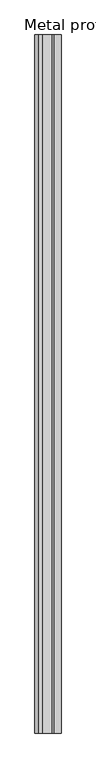
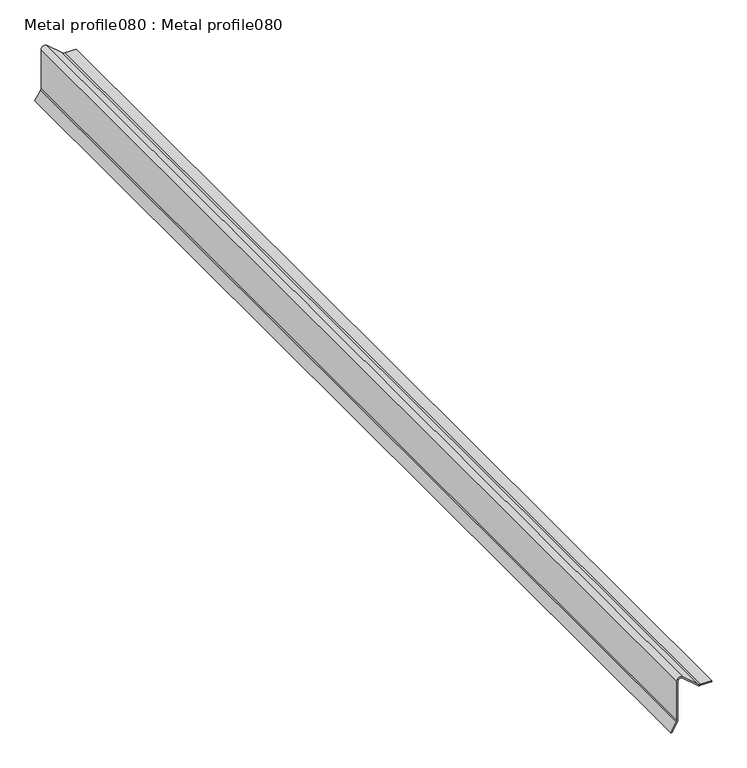
"""IFC4 building model written with IfcOpenShell, lengths in millimetres: proxy geometry, Metal profile080 : Metal profile080."""

from ifc_helpers import new_model, si_unit, point, frame, frame_2d, origin, place, context, project, spatial, polyline, circle_curve, trimmed, segment, composite_curve, outline, extrude, source, transform, mapped, element, save


def metal_profile080_metal_profile080_1098f815(model_context):
    return source(origin(), model_context, "Body", "SweptSolid", [
        extrude(outline(composite_curve([segment(trimmed(circle_curve(frame_2d((40173.6742187, -7212.8179539)), 6.35), [point((40167.3242187, -7212.8179539))], [point((40168.8617194, -7216.9607006))], True, "CARTESIAN"), True, "CONTINUOUS"), segment(polyline([(40168.8617194, -7216.9607006), (40193.006585, -7245.0090359)]), True, "CONTINUOUS"), segment(trimmed(circle_curve(frame_2d((40188.1940856, -7249.1517826)), 6.35), [point((40193.006585, -7245.0090359))], [point((40188.1940856, -7255.5017826))], False, "CARTESIAN"), True, "CONTINUOUS"), segment(polyline([(40188.1940856, -7255.5017826), (40113.9784377, -7255.5017826)]), True, "CONTINUOUS"), segment(trimmed(circle_curve(frame_2d((40113.9784377, -7261.8517826)), 6.35), [point((40113.9784377, -7255.5017826))], [point((40110.6358579, -7256.4527401))], True, "CARTESIAN"), True, "CONTINUOUS"), segment(polyline([(40110.6358579, -7256.4527401), (40093.8632812, -7266.8367435), (40092.8105002, -7265.1362577), (40109.5830768, -7254.7522542)]), True, "CONTINUOUS"), segment(trimmed(circle_curve(frame_2d((40113.9784377, -7261.8517826)), 8.35), [point((40109.5830768, -7254.7522542))], [point((40113.9784377, -7253.5017826))], False, "CARTESIAN"), True, "CONTINUOUS"), segment(polyline([(40113.9784377, -7253.5017826), (40188.1940856, -7253.5017826)]), True, "CONTINUOUS"), segment(trimmed(circle_curve(frame_2d((40188.1940856, -7249.1517826)), 4.35), [point((40188.1940856, -7253.5017826))], [point((40191.4908371, -7246.313838))], True, "CARTESIAN"), True, "CONTINUOUS"), segment(polyline([(40191.4908371, -7246.313838), (40167.3459716, -7218.2655027)]), True, "CONTINUOUS"), segment(trimmed(circle_curve(frame_2d((40173.6742187, -7212.8179539)), 8.35), [point((40167.3459716, -7218.2655027))], [point((40165.3242187, -7212.8179539))], False, "CARTESIAN"), True, "CONTINUOUS"), segment(polyline([(40165.3242187, -7212.8179539), (40165.3242188, -7191.8504154), (40167.3242187, -7191.8504154), (40167.3242187, -7212.8179539)]), True, "CONTINUOUS")], self_intersect=False)), frame((0.0, 7982.1531721, 0.0), z_axis=(0.0, 1.0, 0.0), x_axis=(0.0, 0.0, 1.0)), (0.0, 0.0, 1.0), 2000.0),
    ])


if __name__ == "__main__":
    model = new_model("IFC4")
    model_context = context("Model", 3, world=origin())
    ifc_project = project(units=[si_unit("LENGTHUNIT", "METRE", prefix="MILLI")], contexts=[model_context])
    site = spatial("IfcSite", under=ifc_project)
    building = spatial("IfcBuilding", under=site)
    placement = place(None, origin())
    metal_profile080_metal_profile080_shape = metal_profile080_metal_profile080_1098f815(model_context)
    element("IfcBuildingElementProxy", 1, Name="Metal profile080 : Metal profile080", ObjectType="Metal profile080 : Metal profile080", at=placement, inside=building, context=model_context, shape_type="MappedRepresentation", body=[
        mapped(metal_profile080_metal_profile080_shape, transform((0.0, 0.0, 0.0), x_axis=(1.0, 0.0, 0.0), y_axis=(0.0, 1.0, 0.0), z_axis=(0.0, 0.0, 1.0))),
    ])
    save(model, "model.ifc")

# Revit data of these elements
# Type "Metal profile080 : Metal profile080"
#   NameOverride = "Metal profile080"
# Element 1 (IfcBuildingElementProxy, "Metal profile080 : Metal profile080")
#   Materials on its faces: "ANGLE TRIM"
# Materials
#   "ANGLE TRIM": class "Unassigned", colour RGB 250 255 0, transparency 0
